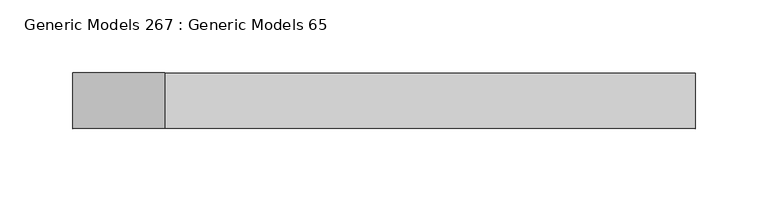
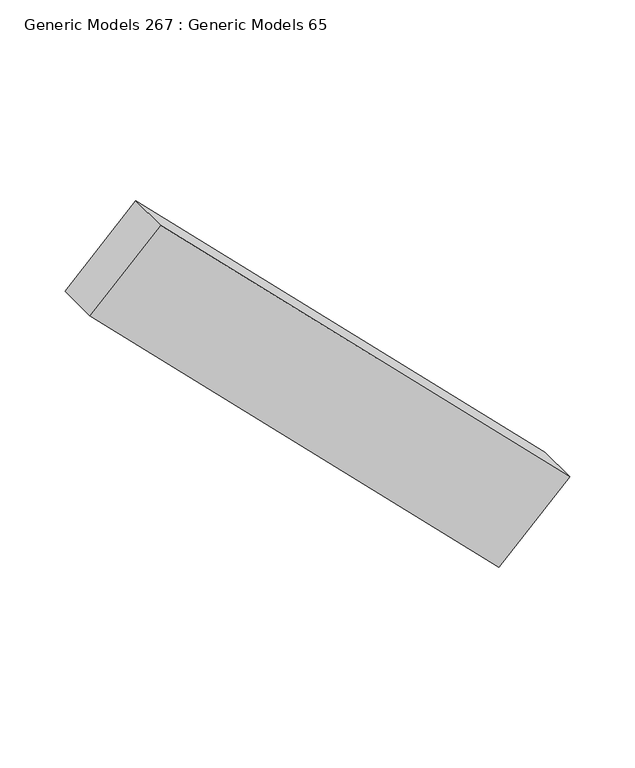
"""IFC4 building model written with IfcOpenShell, lengths in millimetres: proxy geometry, Generic Models 267 : Generic Models 65."""

from ifc_helpers import new_model, si_unit, frame, origin, place, context, project, spatial, polyline, outline, extrude, source, transform, mapped, element, save


def generic_models_267_generic_models_65_11354230(model_context):
    return source(origin(), model_context, "Body", "SweptSolid", [
        extrude(outline(polyline([(0.0, -38.1), (0.0, 0.0), (514.35, 0.0), (514.35, -38.1), (0.0, -38.1)])), frame((47276.4596037, 592.1375, 5202.484661), z_axis=(0.7071067811865633, 0.0, 0.7071067811865317), x_axis=(-0.7071067811865317, 0.0, 0.7071067811865633)), (0.0, 0.0, 1.0), 88.9),
    ])


if __name__ == "__main__":
    model = new_model("IFC4")
    model_context = context("Model", 3, world=origin())
    ifc_project = project(units=[si_unit("LENGTHUNIT", "METRE", prefix="MILLI")], contexts=[model_context])
    site = spatial("IfcSite", under=ifc_project)
    building = spatial("IfcBuilding", under=site)
    placement = place(None, origin())
    generic_models_267_generic_models_65_shape = generic_models_267_generic_models_65_11354230(model_context)
    element("IfcBuildingElementProxy", 1, Name="Generic Models 267 : Generic Models 65", ObjectType="Generic Models 267 : Generic Models 65", at=placement, inside=building, context=model_context, shape_type="MappedRepresentation", body=[
        mapped(generic_models_267_generic_models_65_shape, transform((0.0, 0.0, 0.0), x_axis=(1.0, 0.0, 0.0), y_axis=(0.0, 1.0, 0.0), z_axis=(0.0, 0.0, 1.0))),
    ])
    save(model, "model.ifc")

# Revit data of these elements
# Element 1 (IfcBuildingElementProxy, "Generic Models 267 : Generic Models 65")
#   Materials on its faces: "DIAGONAL BRACING AS REQUIRED"
# Materials
#   "DIAGONAL BRACING AS REQUIRED": class "Wood", colour RGB 234 198 147, transparency 0, Description = "Pinus Echinata", Cost = 0
